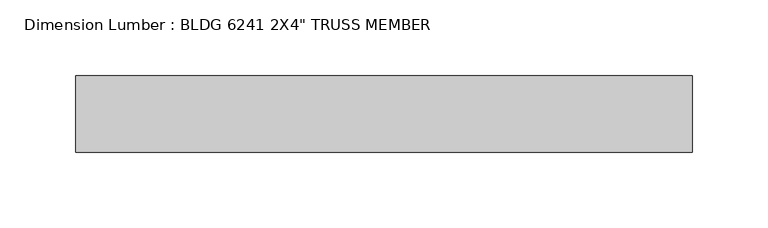
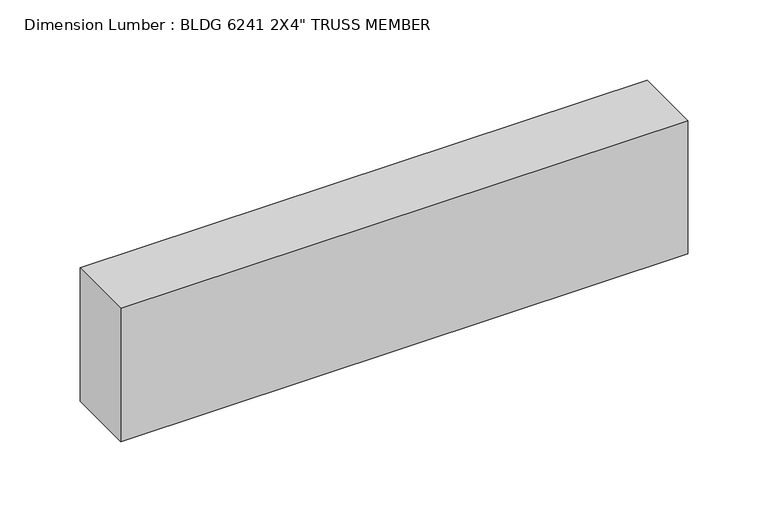
"""IFC4 building model written with IfcOpenShell, lengths in millimetres: beam geometry."""

from ifc_helpers import new_model, si_unit, frame, origin, place, context, project, spatial, polyline, outline, extrude, source, transform, mapped, element, save


def beam_2924e986(model_context):
    return source(origin(), model_context, "Body", "SweptSolid", [
        extrude(outline(polyline([(228.5999994, 25.4), (228.5999994, -25.4), (-179.8629717, -25.4), (-179.8629717, 25.4), (228.5999994, 25.4)])), frame((0.0, 0.0, -50.8), z_axis=(0.0, 0.0, 1.0), x_axis=(1.0, 0.0, 0.0)), (0.0, 0.0, 1.0), 101.6),
    ])


if __name__ == "__main__":
    model = new_model("IFC4")
    model_context = context("Model", 3, world=origin())
    ifc_project = project(units=[si_unit("LENGTHUNIT", "METRE", prefix="MILLI")], contexts=[model_context])
    site = spatial("IfcSite", under=ifc_project)
    building = spatial("IfcBuilding", under=site)
    placement = place(None, origin())
    beam_shape = beam_2924e986(model_context)
    element("IfcBeam", 1, ObjectType="Dimension Lumber : BLDG 6241 2X4\" TRUSS MEMBER", at=placement, inside=building, context=model_context, shape_type="MappedRepresentation", body=[
        mapped(beam_shape, transform((0.0, 0.0, 0.0), x_axis=(1.0, 0.0, 0.0), y_axis=(0.0, 1.0, 0.0), z_axis=(0.0, 0.0, 1.0))),
    ])
    save(model, "model.ifc")

# Revit data of these elements
# Type "Dimension Lumber : BLDG 6241 2X4\" TRUSS MEMBER"
#   Assembly Code = "B10"
#   A = 0.273472 SF
#   Length [instance default] = 5' - 0"
#   b = 0' - 2"
#   d = 0' - 4"
#   Structural Material [instance default] = Softwood, Lumber
# Element 1 (IfcBeam, "Dimension Lumber : BLDG 6241 2X4\" TRUSS MEMBER")
#   Materials on its faces: "Softwood, Lumber"
# Materials
#   "Softwood, Lumber": class "Wood", colour RGB 223 192 134, transparency 0, Description = "Pinus Echinata", Cost = 0
